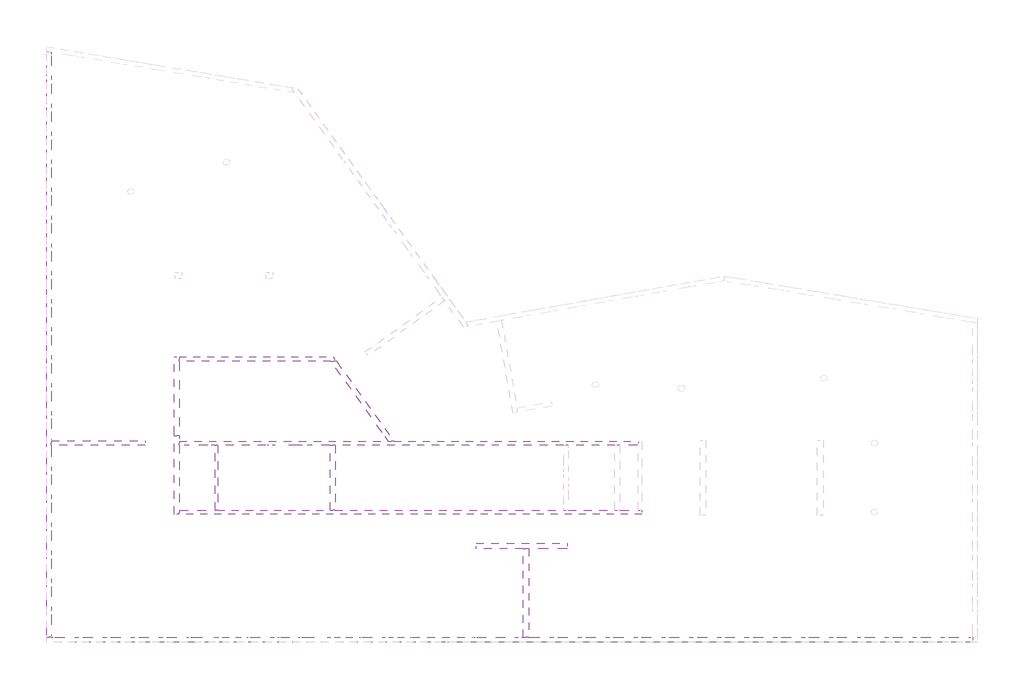
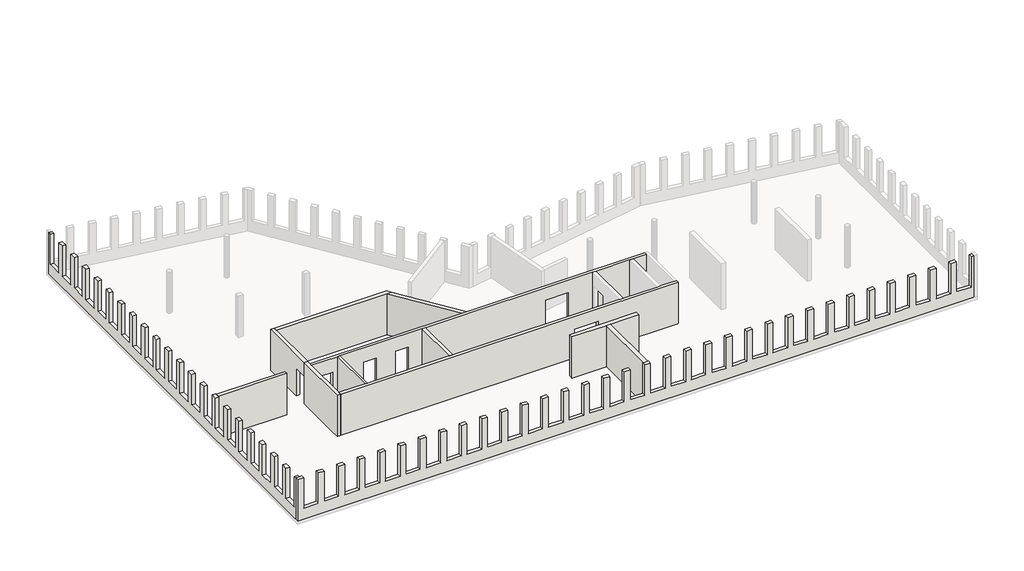
# One storey, part 1 of 2: 13 walls.
"""IFC4 building model written with IfcOpenShell, lengths in millimetres."""

from ifc_helpers import new_model, si_unit, frame, origin, place, context, project, spatial, polyline, outline, extrude, faceted_brep, element, save

model = new_model("IFC4")

# Units and contexts
model_context = context("Model", 3, world=origin())
ifc_project = project(units=[si_unit("LENGTHUNIT", "METRE", prefix="MILLI")], contexts=[model_context])

# Site, building, storey
site = spatial("IfcSite", under=ifc_project)
building = spatial("IfcBuilding", under=site)
storey = spatial("IfcBuildingStorey", under=building, Name="03_OG_OKFB_10,38", Elevation=10380.0)

# Walls
placement = place(None, origin())
element("IfcWall", 1, ObjectType="5dki Lochfassade 26cm C30/37", at=placement, inside=storey, context=model_context, shape_type="Brep", body=[
    faceted_brep([(49396.9999991, 130.0010483, 14550.0), (49396.9999991, 130.0010483, 16900.0), (49603.9991101, 130.0010486, 16900.0), (49603.9991101, 130.0010486, 13690.0), (25766.9999915, 130.0010117, 13690.0), (25466.9999915, 130.0010113, 13690.0), (130.0010047, 130.000972, 13690.0), (-129.9989953, 130.0009716, 13690.0), (-129.9989953, 130.0009716, 16900.0), (130.0010047, 130.000972, 16900.0), (317.0000012, 130.0009723, 16900.0), (316.999997, 130.0009723, 14550.0), (1397.0000012, 130.000974, 14550.0), (1397.0000069, 130.000974, 16900.0), (1816.9999991, 130.0009747, 16900.0), (1817.0000028, 130.0009747, 14550.0), (2896.9999991, 130.0009763, 14550.0), (2897.0000017, 130.0009763, 16900.0), (3316.9999991, 130.000977, 16900.0), (3316.9999977, 130.000977, 14550.0), (4396.9999991, 130.0009787, 14550.0), (4396.9999966, 130.0009787, 16900.0), (4816.9999991, 130.0009793, 16900.0), (4816.9999991, 130.0009793, 14550.0), (5896.9999991, 130.000981, 14550.0), (5896.9999991, 130.000981, 16900.0), (6316.9999991, 130.0009816, 16900.0), (6316.9999991, 130.0009816, 14550.0), (7396.9999991, 130.0009833, 14550.0), (7396.9999991, 130.0009833, 16900.0), (7816.9999991, 130.0009839, 16900.0), (7816.9999991, 130.0009839, 14550.0), (8896.9999991, 130.0009856, 14550.0), (8896.9999991, 130.0009856, 16900.0), (9316.9999991, 130.0009863, 16900.0), (9316.9999991, 130.0009863, 14550.0), (10396.9999991, 130.0009879, 14550.0), (10396.9999991, 130.0009879, 16900.0), (10816.9999991, 130.0009886, 16900.0), (10816.9999991, 130.0009886, 14550.0), (11896.9999991, 130.0009903, 14550.0), (11896.9999991, 130.0009903, 16900.0), (12316.9999991, 130.0009909, 16900.0), (12316.9999991, 130.0009909, 14550.0), (13396.9999991, 130.0009926, 14550.0), (13396.9999991, 130.0009926, 16900.0), (13816.9999991, 130.0009932, 16900.0), (13816.9999991, 130.0009932, 14550.0), (14896.9999991, 130.0009949, 14550.0), (14896.9999991, 130.0009949, 16900.0), (15316.9999991, 130.0009956, 16900.0), (15316.9999991, 130.0009956, 14550.0), (16396.9999991, 130.0009972, 14550.0), (16396.9999991, 130.0009972, 16900.0), (16816.9999991, 130.0009979, 16900.0), (16816.9999991, 130.0009979, 14550.0), (17896.9999991, 130.0009996, 14550.0), (17896.9999991, 130.0009996, 16900.0), (18316.9999991, 130.0010002, 16900.0), (18316.9999991, 130.0010002, 14550.0), (19396.9999991, 130.0010019, 14550.0), (19396.9999991, 130.0010019, 16900.0), (19816.9999991, 130.0010025, 16900.0), (19816.9999991, 130.0010025, 14550.0), (20896.9999991, 130.0010042, 14550.0), (20896.9999991, 130.0010042, 16900.0), (21316.9999991, 130.0010048, 16900.0), (21316.9999991, 130.0010048, 14550.0), (22396.9999991, 130.0010065, 14550.0), (22396.9999991, 130.0010065, 16900.0), (22816.9999991, 130.0010072, 16900.0), (22816.9999991, 130.0010072, 14550.0), (23896.9999991, 130.0010088, 14550.0), (23896.9999991, 130.0010088, 16900.0), (24316.9999991, 130.0010095, 16900.0), (24316.9999991, 130.0010095, 14550.0), (25396.9999991, 130.0010112, 14550.0), (25396.9999991, 130.0010112, 16900.0), (25466.9999915, 130.0010113, 16900.0), (25766.9999915, 130.0010117, 16900.0), (25816.9999991, 130.0010118, 16900.0), (25816.9999991, 130.0010118, 14550.0), (26896.9999991, 130.0010135, 14550.0), (26896.9999991, 130.0010135, 16900.0), (27316.9999991, 130.0010141, 16900.0), (27316.9999991, 130.0010141, 14550.0), (28396.9999991, 130.0010158, 14550.0), (28396.9999991, 130.0010158, 16900.0), (28816.9999991, 130.0010165, 16900.0), (28816.9999991, 130.0010165, 14550.0), (29896.9999991, 130.0010181, 14550.0), (29896.9999991, 130.0010181, 16900.0), (30316.9999991, 130.0010188, 16900.0), (30316.9999991, 130.0010188, 14550.0), (31396.9999991, 130.0010205, 14550.0), (31396.9999991, 130.0010205, 16900.0), (31816.9999991, 130.0010211, 16900.0), (31816.9999991, 130.0010211, 14550.0), (32896.9999991, 130.0010228, 14550.0), (32896.9999991, 130.0010228, 16900.0), (33316.9999991, 130.0010234, 16900.0), (33316.9999991, 130.0010234, 14550.0), (34396.9999991, 130.0010251, 14550.0), (34396.9999991, 130.0010251, 16900.0), (34816.9999991, 130.0010258, 16900.0), (34816.9999991, 130.0010258, 14550.0), (35896.9999991, 130.0010274, 14550.0), (35896.9999991, 130.0010274, 16900.0), (36316.9999991, 130.0010281, 16900.0), (36316.9999991, 130.0010281, 14550.0), (37396.9999991, 130.0010297, 14550.0), (37396.9999991, 130.0010297, 16900.0), (37816.9999991, 130.0010304, 16900.0), (37816.9999991, 130.0010304, 14550.0), (38896.9999991, 130.0010321, 14550.0), (38896.9999991, 130.0010321, 16900.0), (39316.9999991, 130.0010327, 16900.0), (39316.9999991, 130.0010327, 14550.0), (40396.9999991, 130.0010344, 14550.0), (40396.9999991, 130.0010344, 16900.0), (40816.9999991, 130.001035, 16900.0), (40816.9999991, 130.001035, 14550.0), (41896.9999991, 130.0010367, 14550.0), (41896.9999991, 130.0010367, 16900.0), (42316.9999991, 130.0010374, 16900.0), (42316.9999991, 130.0010374, 14550.0), (43396.9999991, 130.001039, 14550.0), (43396.9999991, 130.001039, 16900.0), (43816.9999991, 130.0010397, 16900.0), (43816.9999991, 130.0010397, 14550.0), (44896.9999991, 130.0010414, 14550.0), (44896.9999991, 130.0010414, 16900.0), (45316.9999991, 130.001042, 16900.0), (45316.9999991, 130.001042, 14550.0), (46396.9999991, 130.0010437, 14550.0), (46396.9999991, 130.0010437, 16900.0), (46816.9999991, 130.0010443, 16900.0), (46816.9999991, 130.0010443, 14550.0), (47896.9999991, 130.001046, 14550.0), (47896.9999991, 130.001046, 16900.0), (48316.9999991, 130.0010467, 16900.0), (48316.9999991, 130.0010467, 14550.0), (49603.9991105, -129.9989514, 16900.0), (49396.9999995, -129.9989517, 16900.0), (49396.9999995, -129.9989517, 14550.0), (48316.9999995, -129.9989533, 14550.0), (48316.9999995, -129.9989533, 16900.0), (47896.9999995, -129.998954, 16900.0), (47896.9999995, -129.998954, 14550.0), (46816.9999995, -129.9989557, 14550.0), (46816.9999995, -129.9989557, 16900.0), (46396.9999995, -129.9989563, 16900.0), (46396.9999995, -129.9989563, 14550.0), (45316.9999995, -129.998958, 14550.0), (45316.9999995, -129.998958, 16900.0), (44896.9999995, -129.9989586, 16900.0), (44896.9999995, -129.9989586, 14550.0), (43816.9999995, -129.9989603, 14550.0), (43816.9999995, -129.9989603, 16900.0), (43396.9999995, -129.998961, 16900.0), (43396.9999995, -129.998961, 14550.0), (42316.9999995, -129.9989626, 14550.0), (42316.9999995, -129.9989626, 16900.0), (41896.9999995, -129.9989633, 16900.0), (41896.9999995, -129.9989633, 14550.0), (40816.9999995, -129.998965, 14550.0), (40816.9999995, -129.998965, 16900.0), (40396.9999995, -129.9989656, 16900.0), (40396.9999995, -129.9989656, 14550.0), (39316.9999995, -129.9989673, 14550.0), (39316.9999995, -129.9989673, 16900.0), (38896.9999995, -129.9989679, 16900.0), (38896.9999995, -129.9989679, 14550.0), (37816.9999995, -129.9989696, 14550.0), (37816.9999995, -129.9989696, 16900.0), (37396.9999995, -129.9989703, 16900.0), (37396.9999995, -129.9989703, 14550.0), (36316.9999995, -129.9989719, 14550.0), (36316.9999995, -129.9989719, 16900.0), (35896.9999995, -129.9989726, 16900.0), (35896.9999995, -129.9989726, 14550.0), (34816.9999995, -129.9989742, 14550.0), (34816.9999995, -129.9989742, 16900.0), (34396.9999995, -129.9989749, 16900.0), (34396.9999995, -129.9989749, 14550.0), (33316.9999995, -129.9989766, 14550.0), (33316.9999995, -129.9989766, 16900.0), (32896.9999995, -129.9989772, 16900.0), (32896.9999995, -129.9989772, 14550.0), (31816.9999995, -129.9989789, 14550.0), (31816.9999995, -129.9989789, 16900.0), (31396.9999995, -129.9989795, 16900.0), (31396.9999995, -129.9989795, 14550.0), (30316.9999995, -129.9989812, 14550.0), (30316.9999995, -129.9989812, 16900.0), (29896.9999995, -129.9989819, 16900.0), (29896.9999995, -129.9989819, 14550.0), (28816.9999995, -129.9989835, 14550.0), (28816.9999995, -129.9989835, 16900.0), (28396.9999995, -129.9989842, 16900.0), (28396.9999995, -129.9989842, 14550.0), (27316.9999995, -129.9989859, 14550.0), (27316.9999995, -129.9989859, 16900.0), (26896.9999995, -129.9989865, 16900.0), (26896.9999995, -129.9989865, 14550.0), (25816.9999995, -129.9989882, 14550.0), (25816.9999995, -129.9989882, 16900.0), (25396.9999995, -129.9989888, 16900.0), (25396.9999995, -129.9989888, 14550.0), (24316.9999995, -129.9989905, 14550.0), (24316.9999995, -129.9989905, 16900.0), (23896.9999995, -129.9989912, 16900.0), (23896.9999995, -129.9989912, 14550.0), (22816.9999995, -129.9989928, 14550.0), (22816.9999995, -129.9989928, 16900.0), (22396.9999995, -129.9989935, 16900.0), (22396.9999995, -129.9989935, 14550.0), (21316.9999995, -129.9989952, 14550.0), (21316.9999995, -129.9989952, 16900.0), (20896.9999995, -129.9989958, 16900.0), (20896.9999995, -129.9989958, 14550.0), (19816.9999995, -129.9989975, 14550.0), (19816.9999995, -129.9989975, 16900.0), (19396.9999995, -129.9989981, 16900.0), (19396.9999995, -129.9989981, 14550.0), (18316.9999995, -129.9989998, 14550.0), (18316.9999995, -129.9989998, 16900.0), (17896.9999995, -129.9990004, 16900.0), (17896.9999995, -129.9990004, 14550.0), (16816.9999995, -129.9990021, 14550.0), (16816.9999995, -129.9990021, 16900.0), (16396.9999995, -129.9990028, 16900.0), (16396.9999995, -129.9990028, 14550.0), (15316.9999995, -129.9990044, 14550.0), (15316.9999995, -129.9990044, 16900.0), (14896.9999995, -129.9990051, 16900.0), (14896.9999995, -129.9990051, 14550.0), (13816.9999995, -129.9990068, 14550.0), (13816.9999995, -129.9990068, 16900.0), (13396.9999995, -129.9990074, 16900.0), (13396.9999995, -129.9990074, 14550.0), (12316.9999995, -129.9990091, 14550.0), (12316.9999995, -129.9990091, 16900.0), (11896.9999995, -129.9990097, 16900.0), (11896.9999995, -129.9990097, 14550.0), (10816.9999995, -129.9990114, 14550.0), (10816.9999995, -129.9990114, 16900.0), (10396.9999995, -129.9990121, 16900.0), (10396.9999995, -129.9990121, 14550.0), (9316.9999995, -129.9990137, 14550.0), (9316.9999995, -129.9990137, 16900.0), (8896.9999995, -129.9990144, 16900.0), (8896.9999995, -129.9990144, 14550.0), (7816.9999995, -129.9990161, 14550.0), (7816.9999995, -129.9990161, 16900.0), (7396.9999995, -129.9990167, 16900.0), (7396.9999995, -129.9990167, 14550.0), (6316.9999995, -129.9990184, 14550.0), (6316.9999995, -129.9990184, 16900.0), (5896.9999995, -129.999019, 16900.0), (5896.9999995, -129.999019, 14550.0), (4816.9999995, -129.9990207, 14550.0), (4816.9999995, -129.9990207, 16900.0), (4396.9999995, -129.9990213, 16900.0), (4396.9999966, -129.9990213, 14550.0), (3316.9999995, -129.999023, 14550.0), (3316.9999977, -129.999023, 16900.0), (2896.9999995, -129.9990237, 16900.0), (2897.0000017, -129.9990237, 14550.0), (1816.9999995, -129.9990253, 14550.0), (1817.0000028, -129.9990253, 16900.0), (1397.0000016, -129.999026, 16900.0), (1397.0000069, -129.999026, 14550.0), (317.0000016, -129.9990277, 14550.0), (316.999997, -129.9990277, 16900.0), (-129.9989953, -129.9990284, 16900.0), (-129.9989953, -129.9990284, 13690.0), (49603.9991105, -129.9989514, 13690.0)], [[[0, 1, 2, 3, 4, 5, 6, 7, 8, 9, 10, 11, 12, 13, 14, 15, 16, 17, 18, 19, 20, 21, 22, 23, 24, 25, 26, 27, 28, 29, 30, 31, 32, 33, 34, 35, 36, 37, 38, 39, 40, 41, 42, 43, 44, 45, 46, 47, 48, 49, 50, 51, 52, 53, 54, 55, 56, 57, 58, 59, 60, 61, 62, 63, 64, 65, 66, 67, 68, 69, 70, 71, 72, 73, 74, 75, 76, 77, 78, 79, 80, 81, 82, 83, 84, 85, 86, 87, 88, 89, 90, 91, 92, 93, 94, 95, 96, 97, 98, 99, 100, 101, 102, 103, 104, 105, 106, 107, 108, 109, 110, 111, 112, 113, 114, 115, 116, 117, 118, 119, 120, 121, 122, 123, 124, 125, 126, 127, 128, 129, 130, 131, 132, 133, 134, 135, 136, 137, 138, 139, 140, 141]], [[142, 143, 144, 145, 146, 147, 148, 149, 150, 151, 152, 153, 154, 155, 156, 157, 158, 159, 160, 161, 162, 163, 164, 165, 166, 167, 168, 169, 170, 171, 172, 173, 174, 175, 176, 177, 178, 179, 180, 181, 182, 183, 184, 185, 186, 187, 188, 189, 190, 191, 192, 193, 194, 195, 196, 197, 198, 199, 200, 201, 202, 203, 204, 205, 206, 207, 208, 209, 210, 211, 212, 213, 214, 215, 216, 217, 218, 219, 220, 221, 222, 223, 224, 225, 226, 227, 228, 229, 230, 231, 232, 233, 234, 235, 236, 237, 238, 239, 240, 241, 242, 243, 244, 245, 246, 247, 248, 249, 250, 251, 252, 253, 254, 255, 256, 257, 258, 259, 260, 261, 262, 263, 264, 265, 266, 267, 268, 269, 270, 271, 272, 273, 274, 275, 276, 277]], [[7, 6, 5, 4, 3, 277, 276]], [[17, 267, 266, 18]], [[270, 14, 13, 271]], [[263, 262, 22, 21]], [[259, 258, 26, 25]], [[255, 254, 30, 29]], [[251, 250, 34, 33]], [[247, 246, 38, 37]], [[243, 242, 42, 41]], [[239, 238, 46, 45]], [[235, 234, 50, 49]], [[231, 230, 54, 53]], [[227, 226, 58, 57]], [[223, 222, 62, 61]], [[219, 218, 66, 65]], [[215, 214, 70, 69]], [[211, 210, 74, 73]], [[207, 206, 80, 79, 78, 77]], [[203, 202, 84, 83]], [[199, 198, 88, 87]], [[195, 194, 92, 91]], [[191, 190, 96, 95]], [[187, 186, 100, 99]], [[183, 182, 104, 103]], [[179, 178, 108, 107]], [[175, 174, 112, 111]], [[171, 170, 116, 115]], [[167, 166, 120, 119]], [[163, 162, 124, 123]], [[159, 158, 128, 127]], [[155, 154, 132, 131]], [[151, 150, 136, 135]], [[140, 139, 147, 146]], [[2, 1, 143, 142]], [[10, 9, 8, 275, 274]], [[3, 2, 142, 277]], [[12, 272, 271, 13]], [[273, 11, 10, 274]], [[272, 12, 11, 273]], [[16, 268, 267, 17]], [[269, 15, 14, 270]], [[268, 16, 15, 269]], [[20, 264, 263, 21]], [[265, 19, 18, 266]], [[264, 20, 19, 265]], [[25, 24, 260, 259]], [[23, 22, 262, 261]], [[24, 23, 261, 260]], [[29, 28, 256, 255]], [[27, 26, 258, 257]], [[28, 27, 257, 256]], [[33, 32, 252, 251]], [[31, 30, 254, 253]], [[32, 31, 253, 252]], [[37, 36, 248, 247]], [[35, 34, 250, 249]], [[36, 35, 249, 248]], [[41, 40, 244, 243]], [[39, 38, 246, 245]], [[40, 39, 245, 244]], [[45, 44, 240, 239]], [[43, 42, 242, 241]], [[44, 43, 241, 240]], [[49, 48, 236, 235]], [[47, 46, 238, 237]], [[48, 47, 237, 236]], [[53, 52, 232, 231]], [[51, 50, 234, 233]], [[52, 51, 233, 232]], [[57, 56, 228, 227]], [[55, 54, 230, 229]], [[56, 55, 229, 228]], [[61, 60, 224, 223]], [[59, 58, 226, 225]], [[60, 59, 225, 224]], [[65, 64, 220, 219]], [[63, 62, 222, 221]], [[64, 63, 221, 220]], [[69, 68, 216, 215]], [[67, 66, 218, 217]], [[68, 67, 217, 216]], [[73, 72, 212, 211]], [[71, 70, 214, 213]], [[72, 71, 213, 212]], [[77, 76, 208, 207]], [[75, 74, 210, 209]], [[76, 75, 209, 208]], [[83, 82, 204, 203]], [[81, 80, 206, 205]], [[82, 81, 205, 204]], [[87, 86, 200, 199]], [[85, 84, 202, 201]], [[86, 85, 201, 200]], [[91, 90, 196, 195]], [[89, 88, 198, 197]], [[90, 89, 197, 196]], [[95, 94, 192, 191]], [[93, 92, 194, 193]], [[94, 93, 193, 192]], [[99, 98, 188, 187]], [[97, 96, 190, 189]], [[98, 97, 189, 188]], [[103, 102, 184, 183]], [[101, 100, 186, 185]], [[102, 101, 185, 184]], [[107, 106, 180, 179]], [[105, 104, 182, 181]], [[106, 105, 181, 180]], [[111, 110, 176, 175]], [[109, 108, 178, 177]], [[110, 109, 177, 176]], [[115, 114, 172, 171]], [[113, 112, 174, 173]], [[114, 113, 173, 172]], [[119, 118, 168, 167]], [[117, 116, 170, 169]], [[118, 117, 169, 168]], [[123, 122, 164, 163]], [[121, 120, 166, 165]], [[122, 121, 165, 164]], [[127, 126, 160, 159]], [[125, 124, 162, 161]], [[126, 125, 161, 160]], [[131, 130, 156, 155]], [[129, 128, 158, 157]], [[130, 129, 157, 156]], [[135, 134, 152, 151]], [[133, 132, 154, 153]], [[134, 133, 153, 152]], [[139, 138, 148, 147]], [[137, 136, 150, 149]], [[138, 137, 149, 148]], [[146, 145, 141, 140]], [[144, 143, 1, 0]], [[145, 144, 0, 141]], [[8, 7, 276, 275]]]),
])
element("IfcWall", 2, ObjectType="5dki STB-Wand Kern 25cm C30/37", at=placement, inside=storey, context=model_context, shape_type="Brep", body=[
    faceted_brep([(6989.9999766, 15192.0124447, 16900.0), (6989.9999766, 14942.0124447, 16900.0), (6989.9999766, 10947.0136187, 16900.0), (6989.9999766, 10947.0136187, 15825.0), (6989.9999766, 11957.013616, 15825.0), (6989.9999766, 11957.013616, 13690.0), (6989.9999766, 14942.0124447, 13690.0), (6989.9999766, 15192.0124447, 13690.0), (6739.9999766, 10947.0136187, 16900.0), (6739.9999766, 15192.0124447, 16900.0), (6739.9999766, 15192.0124447, 13690.0), (6739.9999766, 11957.013616, 13690.0), (6739.9999766, 11957.013616, 15825.0), (6739.9999766, 10947.0136187, 15825.0)], [[[0, 1, 2, 3, 4, 5, 6, 7]], [[8, 9, 10, 11, 12, 13]], [[10, 7, 6, 5, 11]], [[2, 1, 0, 9, 8]], [[2, 8, 13, 3]], [[0, 7, 10, 9]], [[4, 12, 11, 5]], [[12, 4, 3, 13]]]),
])
element("IfcWall", 3, ObjectType="5dki STB-Wand Kern 25cm C30/37", at=placement, inside=storey, context=model_context, shape_type="Brep", body=[
    faceted_brep([(6989.9999766, 14942.0124447, 13690.0), (15141.8279932, 14942.0124447, 13690.0), (15449.8792779, 14942.0124447, 13690.0), (15449.8792779, 14942.0124447, 16900.0), (15141.8279932, 14942.0124447, 16900.0), (6989.9999766, 14942.0124447, 16900.0), (6989.9999766, 15192.0124447, 13690.0), (6989.9999766, 15192.0124447, 16900.0), (15269.8915173, 15192.0124447, 16900.0), (15269.8915173, 15192.0124447, 13690.0)], [[[0, 1, 2, 3, 4, 5]], [[6, 7, 8, 9]], [[2, 1, 0, 6, 9]], [[5, 4, 3, 8, 7]], [[0, 5, 7, 6]], [[3, 2, 9, 8]]]),
])
element("IfcWall", 4, ObjectType="5dki STB-Wand Kern 25cm C30/37", at=placement, inside=storey, context=model_context, shape_type="Brep", body=[
    faceted_brep([(18223.2182524, 10662.0127257, 16900.0), (15141.8279932, 14942.0124447, 16900.0), (15141.8279932, 14942.0124447, 13690.0), (17305.3310134, 11936.9428041, 13690.0), (17305.3310134, 11936.9428041, 15825.0), (17895.4523577, 11117.2740911, 15825.0), (17895.4523577, 11117.2740911, 13690.0), (18223.2182524, 10662.0127257, 13690.0), (15449.8792779, 14942.0124447, 16900.0), (18531.2695366, 10662.0127262, 16900.0), (18531.2695366, 10662.0127262, 13690.0), (18098.340653, 11263.3437308, 13690.0), (18098.340653, 11263.3437308, 15825.0), (17508.2193087, 12083.0124438, 15825.0), (17508.2193087, 12083.0124438, 13690.0), (15449.8792779, 14942.0124447, 13690.0)], [[[0, 1, 2, 3, 4, 5, 6, 7]], [[8, 9, 10, 11, 12, 13, 14, 15]], [[2, 15, 14, 3]], [[10, 7, 6, 11]], [[1, 0, 9, 8]], [[2, 1, 8, 15]], [[0, 7, 10, 9]], [[13, 4, 3, 14]], [[4, 13, 12, 5]], [[5, 12, 11, 6]]]),
])
element("IfcWall", 5, ObjectType="5dki STB-Wand Kern 25cm C30/37", at=placement, inside=storey, context=model_context, shape_type="Brep", body=[
    faceted_brep([(6739.9995723, 10947.0136187, 13690.0), (6739.9995723, 6740.0000204, 13690.0), (6739.9995723, 6740.0000204, 16900.0), (6739.9995723, 10947.0136187, 16900.0), (6739.9995723, 10947.0136187, 15825.0), (6989.9995723, 10947.0136187, 13690.0), (6989.9995723, 10947.0136187, 15825.0), (6989.9995723, 10947.0136187, 16900.0), (6989.9995723, 10662.0127052, 16900.0), (6989.9995723, 10442.0127052, 16900.0), (6989.9995723, 6960.0000208, 16900.0), (6989.9995723, 6740.0000208, 16900.0), (6989.9995723, 6740.0000208, 13690.0), (6989.9995723, 6960.0000208, 13690.0), (6989.9995723, 10442.0127052, 13690.0), (6989.9995723, 10662.0127052, 13690.0)], [[[0, 1, 2, 3, 4]], [[5, 6, 7, 8, 9, 10, 11, 12, 13, 14, 15]], [[1, 0, 5, 15, 14, 13, 12]], [[3, 2, 11, 10, 9, 8, 7]], [[0, 4, 3, 7, 6, 5]], [[2, 1, 12, 11]]]),
])
element("IfcWall", 6, ObjectType="5dki STB-Wand Kern 22cm C30/37", at=placement, inside=storey, context=model_context, shape_type="Brep", body=[
    faceted_brep([(31841.999935, 6740.0000516, 16900.0), (6989.9995723, 6740.0000208, 16900.0), (6989.9995723, 6740.0000208, 13690.0), (24166.9999591, 6740.0000421, 13690.0), (24166.999888, 6740.0000421, 15950.0), (25926.9999591, 6740.0000443, 15950.0), (25927.000338, 6740.0000443, 13690.0), (31841.999935, 6740.0000516, 13690.0), (6989.9995723, 6960.0000208, 16900.0), (8916.9999886, 6960.0000232, 16900.0), (9066.9999886, 6960.0000233, 16900.0), (15117.0008797, 6960.0000309, 16900.0), (15367.0008797, 6960.0000312, 16900.0), (27641.9999886, 6960.0000464, 16900.0), (27891.9999886, 6960.0000467, 16900.0), (30391.9999891, 6960.0000498, 16900.0), (30641.9999891, 6960.0000501, 16900.0), (31641.9999382, 6960.0000514, 16900.0), (31841.9999382, 6960.0000516, 16900.0), (31841.9999382, 6960.0000516, 13690.0), (31641.9999382, 6960.0000514, 13690.0), (30641.9999891, 6960.0000501, 13690.0), (30391.9999891, 6960.0000498, 13690.0), (27891.9999886, 6960.0000467, 13690.0), (27641.9999886, 6960.0000464, 13690.0), (25926.9999588, 6960.0000443, 13690.0), (25927.000338, 6960.0000443, 15950.0), (24166.9999588, 6960.0000421, 15950.0), (24166.999888, 6960.0000421, 13690.0), (15367.0008797, 6960.0000312, 13690.0), (15117.0008797, 6960.0000309, 13690.0), (9066.9999886, 6960.0000233, 13690.0), (8916.9999886, 6960.0000232, 13690.0), (6989.9995723, 6960.0000208, 13690.0)], [[[0, 1, 2, 3, 4, 5, 6, 7]], [[8, 9, 10, 11, 12, 13, 14, 15, 16, 17, 18, 19, 20, 21, 22, 23, 24, 25, 26, 27, 28, 29, 30, 31, 32, 33]], [[2, 33, 32, 31, 30, 29, 28, 3]], [[19, 7, 6, 25, 24, 23, 22, 21, 20]], [[1, 0, 18, 17, 16, 15, 14, 13, 12, 11, 10, 9, 8]], [[2, 1, 8, 33]], [[0, 7, 19, 18]], [[5, 26, 25, 6]], [[26, 5, 4, 27]], [[27, 4, 3, 28]]]),
])
element("IfcWall", 7, ObjectType="5dki STB-Wand Kern 22cm C30/37", at=placement, inside=storey, context=model_context, shape_type="Brep", body=[
    faceted_brep([(6989.9995723, 10662.0127052, 16900.0), (18223.2182524, 10662.0127257, 16900.0), (18531.2695366, 10662.0127262, 16900.0), (31641.9999912, 10662.0127502, 16900.0), (31641.9999912, 10662.0127502, 13690.0), (25926.999945, 10662.0127397, 13690.0), (25927.0000254, 10662.0127397, 15950.0), (24166.999945, 10662.0127365, 15950.0), (24166.9998144, 10662.0127365, 13690.0), (18531.2695366, 10662.0127262, 13690.0), (18223.2182524, 10662.0127257, 13690.0), (14152.0004935, 10662.0127182, 13690.0), (14152.0007698, 10662.0127182, 15825.0), (13142.0004935, 10662.0127164, 15825.0), (13142.0009721, 10662.0127164, 13690.0), (11796.9999806, 10662.0127139, 13690.0), (11796.9997327, 10662.0127139, 15825.0), (10786.9999806, 10662.0127121, 15825.0), (10786.999935, 10662.0127121, 13690.0), (8540.0010342, 10662.012708, 13690.0), (8540.000485, 10662.012708, 15825.0), (7530.0010342, 10662.0127061, 15825.0), (7530.0006873, 10662.0127061, 13690.0), (6989.9995723, 10662.0127052, 13690.0), (31641.9999881, 10442.0127502, 16900.0), (30641.9999891, 10442.0127483, 16900.0), (30391.9999891, 10442.0127479, 16900.0), (27891.9999829, 10442.0127433, 16900.0), (27641.9999829, 10442.0127429, 16900.0), (15367.0008797, 10442.0127204, 16900.0), (15117.0008797, 10442.01272, 16900.0), (9066.9999886, 10442.0127089, 16900.0), (8916.9999886, 10442.0127087, 16900.0), (6989.9995723, 10442.0127052, 16900.0), (6989.9995723, 10442.0127052, 13690.0), (7530.0010346, 10442.0127061, 13690.0), (7530.0006873, 10442.0127061, 15825.0), (8540.0010346, 10442.012708, 15825.0), (8540.000485, 10442.012708, 13690.0), (8916.9999886, 10442.0127087, 13690.0), (9066.9999886, 10442.0127089, 13690.0), (10786.999981, 10442.0127121, 13690.0), (10786.999935, 10442.0127121, 15825.0), (11796.999981, 10442.0127139, 15825.0), (11796.9997327, 10442.0127139, 13690.0), (13142.0004939, 10442.0127164, 13690.0), (13142.0009721, 10442.0127164, 15825.0), (14152.0004939, 10442.0127182, 15825.0), (14152.0007698, 10442.0127182, 13690.0), (15117.0008797, 10442.01272, 13690.0), (15367.0008797, 10442.0127204, 13690.0), (24166.9999454, 10442.0127365, 13690.0), (24166.9998144, 10442.0127365, 15950.0), (25926.9999454, 10442.0127397, 15950.0), (25927.0000254, 10442.0127397, 13690.0), (27641.9999829, 10442.0127429, 13690.0), (27891.9999829, 10442.0127433, 13690.0), (30391.9999891, 10442.0127479, 13690.0), (30641.9999891, 10442.0127483, 13690.0), (31641.9999881, 10442.0127502, 13690.0)], [[[0, 1, 2, 3, 4, 5, 6, 7, 8, 9, 10, 11, 12, 13, 14, 15, 16, 17, 18, 19, 20, 21, 22, 23]], [[24, 25, 26, 27, 28, 29, 30, 31, 32, 33, 34, 35, 36, 37, 38, 39, 40, 41, 42, 43, 44, 45, 46, 47, 48, 49, 50, 51, 52, 53, 54, 55, 56, 57, 58, 59]], [[34, 23, 22, 35]], [[4, 59, 58, 57, 56, 55, 54, 5]], [[8, 51, 50, 49, 48, 11, 10, 9]], [[18, 41, 40, 39, 38, 19]], [[44, 15, 14, 45]], [[3, 2, 1, 0, 33, 32, 31, 30, 29, 28, 27, 26, 25, 24]], [[0, 23, 34, 33]], [[4, 3, 24, 59]], [[53, 6, 5, 54]], [[6, 53, 52, 7]], [[7, 52, 51, 8]], [[17, 42, 41, 18]], [[42, 17, 16, 43]], [[43, 16, 15, 44]], [[13, 46, 45, 14]], [[46, 13, 12, 47]], [[47, 12, 11, 48]], [[21, 36, 35, 22]], [[36, 21, 20, 37]], [[37, 20, 19, 38]]]),
])
element("IfcWall", 8, ObjectType="5dki STB-Wand Kern 25cm C30/37", at=placement, inside=storey, context=model_context, shape_type="SweptSolid", body=[
    extrude(outline(polyline([(15117.0008797, 6960.0000309), (15117.0008797, 10442.01272), (15367.0008797, 10442.0127204), (15367.0008797, 6960.0000312), (15117.0008797, 6960.0000309)])), frame((0.0, 0.0, 13690.0), z_axis=(0.0, 0.0, 1.0), x_axis=(1.0, 0.0, 0.0)), (0.0, 0.0, 1.0), 3210.0),
])
element("IfcWall", 9, ObjectType="5dki STB-Wand Kern 15cm C30/37", at=placement, inside=storey, context=model_context, shape_type="SweptSolid", body=[
    extrude(outline(polyline([(8916.9999886, 6960.0000232), (8916.9999886, 10442.0127087), (9066.9999886, 10442.0127089), (9066.9999886, 6960.0000233), (8916.9999886, 6960.0000232)])), frame((0.0, 0.0, 13690.0), z_axis=(0.0, 0.0, 1.0), x_axis=(1.0, 0.0, 0.0)), (0.0, 0.0, 1.0), 3210.0),
])
element("IfcWall", 10, ObjectType="5dki Lochfassade 26cm C30/37", at=placement, inside=storey, context=model_context, shape_type="Brep", body=[
    faceted_brep([(130.0010047, 24278.4322867, 14550.0), (130.0010047, 24278.4322867, 16900.0), (130.0010047, 23857.0124158, 16900.0), (130.0010047, 23857.0124158, 14550.0), (130.0010047, 22777.0124158, 14550.0), (130.0010047, 22777.0124158, 16900.0), (130.0010047, 22357.0124158, 16900.0), (130.0010047, 22357.0124158, 14550.0), (130.0010047, 21277.0124158, 14550.0), (130.0010047, 21277.0124158, 16900.0), (130.0010047, 20857.0124158, 16900.0), (130.0010047, 20857.0124158, 14550.0), (130.0010047, 19777.0124158, 14550.0), (130.0010047, 19777.0124158, 16900.0), (130.0010047, 19357.0124158, 16900.0), (130.0010047, 19357.0124158, 14550.0), (130.0010047, 18277.0124158, 14550.0), (130.0010047, 18277.0124158, 16900.0), (130.0010047, 17857.0124158, 16900.0), (130.0010047, 17857.0124158, 14550.0), (130.0010047, 16777.0124158, 14550.0), (130.0010047, 16777.0124158, 16900.0), (130.0010047, 16357.0124158, 16900.0), (130.0010047, 16357.0124158, 14550.0), (130.0010047, 15277.0124158, 14550.0), (130.0010047, 15277.0124158, 16900.0), (130.0010047, 14857.0124158, 16900.0), (130.0010047, 14857.0124158, 14550.0), (130.0010047, 13777.0124158, 14550.0), (130.0010047, 13777.0124158, 16900.0), (130.0010047, 13357.0124158, 16900.0), (130.0010047, 13357.0124158, 14550.0), (130.0010047, 12277.0124158, 14550.0), (130.0010047, 12277.0124158, 16900.0), (130.0010047, 11857.0124158, 16900.0), (130.0010047, 11857.0124158, 14550.0), (130.0010047, 10777.0124158, 14550.0), (130.0010047, 10777.0124158, 16900.0), (130.0010047, 10692.0124295, 16900.0), (130.0010047, 10442.0124295, 16900.0), (130.0010047, 10357.0124158, 16900.0), (130.0010047, 10357.0124158, 14550.0), (130.0010047, 9277.0124158, 14550.0), (130.0010047, 9277.0124158, 16900.0), (130.0010047, 8857.0124158, 16900.0), (130.0010047, 8857.0124158, 14550.0), (130.0010047, 7777.0124158, 14550.0), (130.0010047, 7777.0124158, 16900.0), (130.0010047, 7357.0124158, 16900.0), (130.0010047, 7357.0124158, 14550.0), (130.0010047, 6277.0124158, 14550.0), (130.0010047, 6277.0124158, 16900.0), (130.0010047, 5857.0124158, 16900.0), (130.0010047, 5857.0124158, 14550.0), (130.0010047, 4777.0124158, 14550.0), (130.0010047, 4777.0124158, 16900.0), (130.0010047, 4357.0124158, 16900.0), (130.0010047, 4357.0124158, 14550.0), (130.0010047, 3277.0124158, 14550.0), (130.0010047, 3277.0124158, 16900.0), (130.0010047, 2857.0124158, 16900.0), (130.0010047, 2857.0124158, 14550.0), (130.0010047, 1777.0124158, 14550.0), (130.0010047, 1777.0124158, 16900.0), (130.0010047, 1357.0124158, 16900.0), (130.0010047, 1357.0124158, 14550.0), (130.0010047, 277.0124158, 14550.0), (130.0010047, 277.0124158, 16900.0), (130.0010047, 130.000972, 16900.0), (130.0010047, 130.000972, 13690.0), (130.0010047, 10442.0124295, 13690.0), (130.0010047, 10692.0124295, 13690.0), (130.0010047, 31548.6978518, 13690.0), (130.0010047, 31548.6978518, 16900.0), (130.0010047, 31357.0124158, 16900.0), (130.0010047, 31357.0124158, 14550.0), (130.0010047, 30277.0124158, 14550.0), (130.0010047, 30277.0124158, 16900.0), (130.0010047, 29857.0124158, 16900.0), (130.0010047, 29857.0124158, 14550.0), (130.0010047, 28777.0124158, 14550.0), (130.0010047, 28777.0124158, 16900.0), (130.0010047, 28358.4322867, 16900.0), (130.0010047, 28358.4322867, 14550.0), (130.0010047, 27278.4322867, 14550.0), (130.0010047, 27278.4322867, 16900.0), (130.0010047, 26858.4322867, 16900.0), (130.0010047, 26858.4322867, 14550.0), (130.0010047, 25778.4322867, 14550.0), (130.0010047, 25778.4322867, 16900.0), (130.0010047, 25358.4322867, 16900.0), (130.0010047, 25358.4322867, 14550.0), (-129.9989953, 23857.0124158, 16900.0), (-129.9989953, 24278.4322867, 16900.0), (-129.9989953, 24278.4322867, 14550.0), (-129.9989953, 25358.4322867, 14550.0), (-129.9989953, 25358.4322867, 16900.0), (-129.9989953, 25778.4322867, 16900.0), (-129.9989953, 25778.4322867, 14550.0), (-129.9989953, 26858.4322867, 14550.0), (-129.9989953, 26858.4322867, 16900.0), (-129.9989953, 27278.4322867, 16900.0), (-129.9989953, 27278.4322867, 14550.0), (-129.9989953, 28358.4322867, 14550.0), (-129.9989953, 28358.4322867, 16900.0), (-129.9989953, 28777.0124158, 16900.0), (-129.9989953, 28777.0124158, 14550.0), (-129.9989953, 29857.0124158, 14550.0), (-129.9989953, 29857.0124158, 16900.0), (-129.9989953, 30277.0124158, 16900.0), (-129.9989953, 30277.0124158, 14550.0), (-129.9989953, 31357.0124158, 14550.0), (-129.9989953, 31357.0124158, 16900.0), (-129.9989953, 31592.114918, 16900.0), (-129.9989953, 31592.114918, 13690.0), (-129.9989953, 130.0009716, 13690.0), (-129.9989953, 130.0009716, 16900.0), (-129.9989953, 277.0124158, 16900.0), (-129.9989953, 277.0124158, 14550.0), (-129.9989953, 1357.0124158, 14550.0), (-129.9989953, 1357.0124158, 16900.0), (-129.9989953, 1777.0124158, 16900.0), (-129.9989953, 1777.0124158, 14550.0), (-129.9989953, 2857.0124158, 14550.0), (-129.9989953, 2857.0124158, 16900.0), (-129.9989953, 3277.0124158, 16900.0), (-129.9989953, 3277.0124158, 14550.0), (-129.9989953, 4357.0124158, 14550.0), (-129.9989953, 4357.0124158, 16900.0), (-129.9989953, 4777.0124158, 16900.0), (-129.9989953, 4777.0124158, 14550.0), (-129.9989953, 5857.0124158, 14550.0), (-129.9989953, 5857.0124158, 16900.0), (-129.9989953, 6277.0124158, 16900.0), (-129.9989953, 6277.0124158, 14550.0), (-129.9989953, 7357.0124158, 14550.0), (-129.9989953, 7357.0124158, 16900.0), (-129.9989953, 7777.0124158, 16900.0), (-129.9989953, 7777.0124158, 14550.0), (-129.9989953, 8857.0124158, 14550.0), (-129.9989953, 8857.0124158, 16900.0), (-129.9989953, 9277.0124158, 16900.0), (-129.9989953, 9277.0124158, 14550.0), (-129.9989953, 10357.0124158, 14550.0), (-129.9989953, 10357.0124158, 16900.0), (-129.9989953, 10777.0124158, 16900.0), (-129.9989953, 10777.0124158, 14550.0), (-129.9989953, 11857.0124158, 14550.0), (-129.9989953, 11857.0124158, 16900.0), (-129.9989953, 12277.0124158, 16900.0), (-129.9989953, 12277.0124158, 14550.0), (-129.9989953, 13357.0124158, 14550.0), (-129.9989953, 13357.0124158, 16900.0), (-129.9989953, 13777.0124158, 16900.0), (-129.9989953, 13777.0124158, 14550.0), (-129.9989953, 14857.0124158, 14550.0), (-129.9989953, 14857.0124158, 16900.0), (-129.9989953, 15277.0124158, 16900.0), (-129.9989953, 15277.0124158, 14550.0), (-129.9989953, 16357.0124158, 14550.0), (-129.9989953, 16357.0124158, 16900.0), (-129.9989953, 16777.0124158, 16900.0), (-129.9989953, 16777.0124158, 14550.0), (-129.9989953, 17857.0124158, 14550.0), (-129.9989953, 17857.0124158, 16900.0), (-129.9989953, 18277.0124158, 16900.0), (-129.9989953, 18277.0124158, 14550.0), (-129.9989953, 19357.0124158, 14550.0), (-129.9989953, 19357.0124158, 16900.0), (-129.9989953, 19777.0124158, 16900.0), (-129.9989953, 19777.0124158, 14550.0), (-129.9989953, 20857.0124158, 14550.0), (-129.9989953, 20857.0124158, 16900.0), (-129.9989953, 21277.0124158, 16900.0), (-129.9989953, 21277.0124158, 14550.0), (-129.9989953, 22357.0124158, 14550.0), (-129.9989953, 22357.0124158, 16900.0), (-129.9989953, 22777.0124158, 16900.0), (-129.9989953, 22777.0124158, 14550.0), (-129.9989953, 23857.0124158, 14550.0), (90.4211678, 31555.307238, 16900.0)], [[[0, 1, 2, 3, 4, 5, 6, 7, 8, 9, 10, 11, 12, 13, 14, 15, 16, 17, 18, 19, 20, 21, 22, 23, 24, 25, 26, 27, 28, 29, 30, 31, 32, 33, 34, 35, 36, 37, 38, 39, 40, 41, 42, 43, 44, 45, 46, 47, 48, 49, 50, 51, 52, 53, 54, 55, 56, 57, 58, 59, 60, 61, 62, 63, 64, 65, 66, 67, 68, 69, 70, 71, 72, 73, 74, 75, 76, 77, 78, 79, 80, 81, 82, 83, 84, 85, 86, 87, 88, 89, 90, 91]], [[92, 93, 94, 95, 96, 97, 98, 99, 100, 101, 102, 103, 104, 105, 106, 107, 108, 109, 110, 111, 112, 113, 114, 115, 116, 117, 118, 119, 120, 121, 122, 123, 124, 125, 126, 127, 128, 129, 130, 131, 132, 133, 134, 135, 136, 137, 138, 139, 140, 141, 142, 143, 144, 145, 146, 147, 148, 149, 150, 151, 152, 153, 154, 155, 156, 157, 158, 159, 160, 161, 162, 163, 164, 165, 166, 167, 168, 169, 170, 171, 172, 173, 174, 175, 176, 177, 178, 179]], [[72, 71, 70, 69, 115, 114]], [[64, 63, 121, 120]], [[60, 59, 125, 124]], [[56, 55, 129, 128]], [[52, 51, 133, 132]], [[48, 47, 137, 136]], [[44, 43, 141, 140]], [[40, 39, 38, 37, 145, 144]], [[34, 33, 149, 148]], [[30, 29, 153, 152]], [[26, 25, 157, 156]], [[22, 21, 161, 160]], [[18, 17, 165, 164]], [[14, 13, 169, 168]], [[10, 9, 173, 172]], [[6, 5, 177, 176]], [[74, 73, 180, 113, 112]], [[78, 77, 109, 108]], [[82, 81, 105, 104]], [[86, 85, 101, 100]], [[90, 89, 97, 96]], [[2, 1, 93, 92]], [[116, 68, 67, 117]], [[119, 65, 64, 120]], [[66, 118, 117, 67]], [[65, 119, 118, 66]], [[124, 123, 61, 60]], [[122, 121, 63, 62]], [[123, 122, 62, 61]], [[128, 127, 57, 56]], [[126, 125, 59, 58]], [[127, 126, 58, 57]], [[132, 131, 53, 52]], [[130, 129, 55, 54]], [[131, 130, 54, 53]], [[136, 135, 49, 48]], [[134, 133, 51, 50]], [[135, 134, 50, 49]], [[140, 139, 45, 44]], [[138, 137, 47, 46]], [[139, 138, 46, 45]], [[144, 143, 41, 40]], [[142, 141, 43, 42]], [[143, 142, 42, 41]], [[148, 147, 35, 34]], [[146, 145, 37, 36]], [[147, 146, 36, 35]], [[152, 151, 31, 30]], [[150, 149, 33, 32]], [[151, 150, 32, 31]], [[156, 155, 27, 26]], [[154, 153, 29, 28]], [[155, 154, 28, 27]], [[160, 159, 23, 22]], [[158, 157, 25, 24]], [[159, 158, 24, 23]], [[164, 163, 19, 18]], [[162, 161, 21, 20]], [[163, 162, 20, 19]], [[168, 167, 15, 14]], [[166, 165, 17, 16]], [[167, 166, 16, 15]], [[172, 171, 11, 10]], [[170, 169, 13, 12]], [[171, 170, 12, 11]], [[176, 175, 7, 6]], [[174, 173, 9, 8]], [[175, 174, 8, 7]], [[92, 179, 3, 2]], [[178, 177, 5, 4]], [[179, 178, 4, 3]], [[112, 111, 75, 74]], [[110, 109, 77, 76]], [[111, 110, 76, 75]], [[108, 107, 79, 78]], [[106, 105, 81, 80]], [[107, 106, 80, 79]], [[104, 103, 83, 82]], [[102, 101, 85, 84]], [[103, 102, 84, 83]], [[100, 99, 87, 86]], [[98, 97, 89, 88]], [[99, 98, 88, 87]], [[96, 95, 91, 90]], [[94, 93, 1, 0]], [[95, 94, 0, 91]], [[69, 68, 116, 115]], [[73, 72, 114, 113, 180]]]),
])
element("IfcWall", 11, ObjectType="5dki STB-Wand 25cm C30/37", at=placement, inside=storey, context=model_context, shape_type="SweptSolid", body=[
    extrude(outline(polyline([(130.0010047, 10692.0124295), (5179.9999831, 10692.0124295), (5179.9999831, 10442.0124295), (130.0010047, 10442.0124295), (130.0010047, 10692.0124295)])), frame((0.0, 0.0, 13690.0), z_axis=(0.0, 0.0, 1.0), x_axis=(1.0, 0.0, 0.0)), (0.0, 0.0, 1.0), 3210.0),
])
element("IfcWall", 12, ObjectType="5dki STB-Wand 30cm C30/37", at=placement, inside=storey, context=model_context, shape_type="Brep", body=[
    faceted_brep([(22936.4905033, 4880.0000432, 13690.0), (25466.9999915, 4880.0000432, 13690.0), (25766.9999915, 4880.0000432, 13690.0), (27842.0010332, 4880.0000432, 13690.0), (27842.0010332, 4880.0000432, 16900.0), (25766.9999915, 4880.0000432, 16900.0), (25466.9999915, 4880.0000432, 16900.0), (22936.4905033, 4880.0000432, 16900.0), (22936.4905033, 5180.0000432, 13690.0), (22936.4905033, 5180.0000432, 16900.0), (27842.0010332, 5180.0000432, 16900.0), (27842.0010332, 5180.0000432, 13690.0)], [[[0, 1, 2, 3, 4, 5, 6, 7]], [[8, 9, 10, 11]], [[3, 2, 1, 0, 8, 11]], [[4, 3, 11, 10]], [[7, 6, 5, 4, 10, 9]], [[0, 7, 9, 8]]]),
])
element("IfcWall", 13, ObjectType="5dki STB-Wand 30cm C30/37", at=placement, inside=storey, context=model_context, shape_type="SweptSolid", body=[
    extrude(outline(polyline([(25466.9999915, 130.0010113), (25466.9999915, 4880.0000432), (25766.9999915, 4880.0000432), (25766.9999915, 130.0010117), (25466.9999915, 130.0010113)])), frame((0.0, 0.0, 13690.0), z_axis=(0.0, 0.0, 1.0), x_axis=(1.0, 0.0, 0.0)), (0.0, 0.0, 1.0), 3210.0),
])

save(model, "model.ifc")

# Revit data of these elements
# Type "5dki Lochfassade 26cm C30/37"
#   Type Comments = ""
#   Description = ""
#   cpiComponentType = "Wall"
#   cpiFitMatchKey = "5D-KI-STB-OB-W-LF"
#   5d Materialgüte = "C35/45"
#   Filter Tragend / Nichttragend = yes
#   5dki WU = no
#   Layers, outside or top first: 0.260 m "5d Beton - Stahlbeton" (function 1)
# Type "5dki STB-Wand Kern 25cm C30/37"
#   Type Comments = ""
#   Description = ""
#   cpiComponentType = "Wall"
#   cpiFitMatchKey = "5D-KI-STB-OB-W-K"
#   5d Materialgüte = "C30/37"
#   Filter Tragend / Nichttragend = yes
#   5dki WU = no
#   Layers, outside or top first: 0.250 m "5d Beton - Stahlbeton" (function 1)
# Type "5dki STB-Wand Kern 22cm C30/37"
#   Type Comments = ""
#   Description = ""
#   cpiComponentType = "Wall"
#   cpiFitMatchKey = "5D-KI-STB-OB-W-K"
#   5d Materialgüte = "C30/37"
#   Filter Tragend / Nichttragend = yes
#   5dki WU = no
#   Layers, outside or top first: 0.220 m "5d Beton - Stahlbeton" (function 1)
# Type "5dki STB-Wand Kern 15cm C30/37"
#   Type Comments = ""
#   Description = ""
#   cpiComponentType = "Wall"
#   cpiFitMatchKey = "5D-KI-STB-OB-W-K"
#   5d Materialgüte = "C30/37"
#   Filter Tragend / Nichttragend = yes
#   5dki WU = no
#   Layers, outside or top first: 0.150 m "5d Beton - Stahlbeton" (function 1)
# Type "5dki STB-Wand 25cm C30/37"
#   Type Comments = ""
#   Description = ""
#   cpiComponentType = "Wall"
#   cpiFitMatchKey = "5D-KI-STB-OB-W"
#   5d Materialgüte = "C30/37"
#   Filter Tragend / Nichttragend = yes
#   5dki WU = no
#   Layers, outside or top first: 0.250 m "5d Beton - Stahlbeton" (function 1)
# Type "5dki STB-Wand 30cm C30/37"
#   Type Comments = ""
#   Description = ""
#   cpiComponentType = "Wall"
#   cpiFitMatchKey = "5D-KI-STB-OB-W"
#   5d Materialgüte = "C30/37"
#   Filter Tragend / Nichttragend = yes
#   5dki WU = no
#   Layers, outside or top first: 0.300 m "5d Beton - Stahlbeton" (function 1)
# Element 1 (IfcWall, "5dki Lochfassade 26cm C30/37")
#   000_080_030_Geschoß = "04_OG"
#   Top Offset = 0.000 m
#   Base Offset = 0.000 m
#   wall height = 3.210 m
#   Phase Created = Neu
#   Base Constraint = 03_OG_OKRD_13,69
#   Top Constraint = 04_OG_UKRD_16,90
#   Materials on its faces: "5d Beton - Stahlbeton"
# Elements 2, 3, 4, 5, 8 (IfcWall, "5dki STB-Wand Kern 25cm C30/37")
#   Comments = ""
#   000_080_030_Geschoß = "04_OG"
#   Top Offset = 0.000 m
#   Base Offset = 0.000 m
#   wall height = 3.210 m
#   Phase Created = Neu
#   Base Constraint = 03_OG_OKRD_13,69
#   Top Constraint = 04_OG_UKRD_16,90
#   Materials on its faces: "5d Beton - Stahlbeton"
# Elements 6, 7 (IfcWall, "5dki STB-Wand Kern 22cm C30/37")
#   Comments = ""
#   000_080_030_Geschoß = "04_OG"
#   Top Offset = 0.000 m
#   Base Offset = 0.000 m
#   wall height = 3.210 m
#   Phase Created = Neu
#   Base Constraint = 03_OG_OKRD_13,69
#   Top Constraint = 04_OG_UKRD_16,90
#   Materials on its faces: "5d Beton - Stahlbeton"
# Element 9 (IfcWall, "5dki STB-Wand Kern 15cm C30/37")
#   Comments = ""
#   000_080_030_Geschoß = "04_OG"
#   Top Offset = 0.000 m
#   Base Offset = 0.000 m
#   wall height = 3.210 m
#   Phase Created = Neu
#   Base Constraint = 03_OG_OKRD_13,69
#   Top Constraint = 04_OG_UKRD_16,90
#   Materials on its faces: "5d Beton - Stahlbeton"
# Element 10 (IfcWall, "5dki Lochfassade 26cm C30/37")
#   Comments = ""
#   000_080_030_Geschoß = "04_OG"
#   Top Offset = 0.000 m
#   Base Offset = 0.000 m
#   wall height = 3.210 m
#   Phase Created = Neu
#   Base Constraint = 03_OG_OKRD_13,69
#   Top Constraint = 04_OG_UKRD_16,90
#   Materials on its faces: "5d Beton - Stahlbeton"
# Element 11 (IfcWall, "5dki STB-Wand 25cm C30/37")
#   Comments = ""
#   000_080_030_Geschoß = "04_OG"
#   Top Offset = 0.000 m
#   Base Offset = 0.000 m
#   wall height = 3.210 m
#   Phase Created = Neu
#   Base Constraint = 03_OG_OKRD_13,69
#   Top Constraint = 04_OG_UKRD_16,90
#   Materials on its faces: "5d Beton - Stahlbeton"
# Element 12 (IfcWall, "5dki STB-Wand 30cm C30/37")
#   Comments = ""
#   000_080_030_Geschoß = "04_OG"
#   Top Offset = 0.000 m
#   Base Offset = 0.000 m
#   wall height = 3.210 m
#   Phase Created = Neu
#   Base Constraint = 03_OG_OKRD_13,69
#   Top Constraint = 04_OG_UKRD_16,90
#   Materials on its faces: "5d Beton - Stahlbeton"
# Element 13 (IfcWall, "5dki STB-Wand 30cm C30/37")
#   000_080_030_Geschoß = "04_OG"
#   Top Offset = 0.000 m
#   Base Offset = 0.000 m
#   wall height = 3.210 m
#   Phase Created = Neu
#   Base Constraint = 03_OG_OKRD_13,69
#   Top Constraint = 04_OG_UKRD_16,90
#   Materials on its faces: "5d Beton - Stahlbeton"
# Materials
#   "5d Beton - Stahlbeton": class "5dki", colour RGB 200 200 200, transparency 0, Cost = 0
